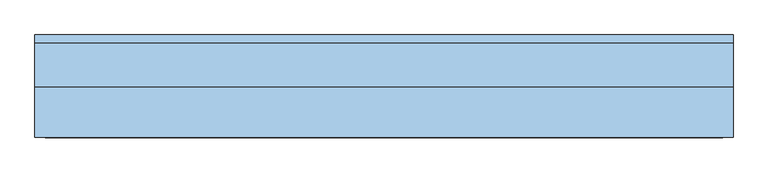
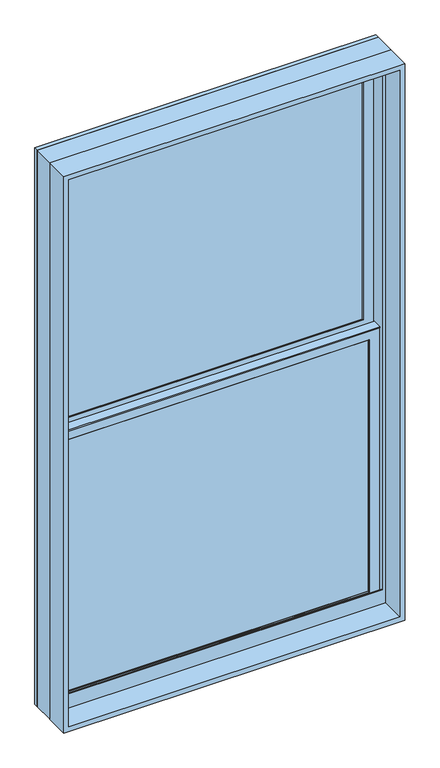
"""IFC4 building model written with IfcOpenShell, lengths in millimetres: window geometry, Window-Double_Hung-Marvin-Essential : ESDH3660."""

from ifc_helpers import new_model, si_unit, frame, origin, place, context, project, spatial, polyline, outline, extrude, faceted_brep, source, transform, mapped, element, save


def window_622c2d66(model_context):
    return source(origin(), model_context, "Body", "SolidModel", [
        extrude(outline(polyline([(166.1583333, 20.6375), (166.1583333, 15.875), (147.1083333, 15.875), (147.1083333, 20.6375), (166.1583333, 20.6375)])), frame((0.0, 0.0, 679.45), z_axis=(0.0, 0.0, 1.0), x_axis=(1.0, 0.0, 0.0)), (0.0, 0.0, 1.0), 831.85),
        extrude(outline(polyline([(-147.1083333, 20.6375), (-147.1083333, 15.875), (-166.1583333, 15.875), (-166.1583333, 20.6375), (-147.1083333, 20.6375)])), frame((0.0, 0.0, 679.45), z_axis=(0.0, 0.0, 1.0), x_axis=(1.0, 0.0, 0.0)), (0.0, 0.0, 1.0), 831.85),
        extrude(outline(polyline([(469.9, 20.6375), (469.9, 15.875), (-469.9, 15.875), (-469.9, 20.6375), (469.9, 20.6375)])), frame((0.0, 0.0, 1085.85), z_axis=(0.0, 0.0, 1.0), x_axis=(1.0, 0.0, 0.0)), (0.0, 0.0, 1.0), 19.05),
        extrude(outline(polyline([(-166.1583333, 46.83125), (-166.1583333, 51.59375), (-147.1083333, 51.59375), (-147.1083333, 46.83125), (-166.1583333, 46.83125)])), frame((0.0, 0.0, 1549.4), z_axis=(0.0, 0.0, 1.0), x_axis=(1.0, 0.0, 0.0)), (0.0, 0.0, 1.0), 831.85),
        extrude(outline(polyline([(147.1083333, 46.83125), (147.1083333, 51.59375), (166.1583333, 51.59375), (166.1583333, 46.83125), (147.1083333, 46.83125)])), frame((0.0, 0.0, 1549.4), z_axis=(0.0, 0.0, 1.0), x_axis=(1.0, 0.0, 0.0)), (0.0, 0.0, 1.0), 831.85),
        extrude(outline(polyline([(-469.9, 46.83125), (-469.9, 51.59375), (469.9, 51.59375), (469.9, 46.83125), (-469.9, 46.83125)])), frame((0.0, 0.0, 1955.8), z_axis=(0.0, 0.0, 1.0), x_axis=(1.0, 0.0, 0.0)), (0.0, 0.0, 1.0), 19.05),
        extrude(outline(polyline([(166.1583333, 20.6375), (147.1083333, 20.6375), (147.1083333, 25.4), (166.1583333, 25.4), (166.1583333, 20.6375)])), frame((0.0, 0.0, 679.45), z_axis=(0.0, 0.0, 1.0), x_axis=(1.0, 0.0, 0.0)), (0.0, 0.0, 1.0), 831.85),
        extrude(outline(polyline([(-147.1083333, 20.6375), (-166.1583333, 20.6375), (-166.1583333, 25.4), (-147.1083333, 25.4), (-147.1083333, 20.6375)])), frame((0.0, 0.0, 679.45), z_axis=(0.0, 0.0, 1.0), x_axis=(1.0, 0.0, 0.0)), (0.0, 0.0, 1.0), 831.85),
        extrude(outline(polyline([(469.9, 20.6375), (-469.9, 20.6375), (-469.9, 25.4), (469.9, 25.4), (469.9, 20.6375)])), frame((0.0, 0.0, 1085.85), z_axis=(0.0, 0.0, 1.0), x_axis=(1.0, 0.0, 0.0)), (0.0, 0.0, 1.0), 19.05),
        extrude(outline(polyline([(-166.1583333, 56.35625), (-147.1083333, 56.35625), (-147.1083333, 51.59375), (-166.1583333, 51.59375), (-166.1583333, 56.35625)])), frame((0.0, 0.0, 1549.4), z_axis=(0.0, 0.0, 1.0), x_axis=(1.0, 0.0, 0.0)), (0.0, 0.0, 1.0), 831.85),
        extrude(outline(polyline([(147.1083333, 56.35625), (166.1583333, 56.35625), (166.1583333, 51.59375), (147.1083333, 51.59375), (147.1083333, 56.35625)])), frame((0.0, 0.0, 1549.4), z_axis=(0.0, 0.0, 1.0), x_axis=(1.0, 0.0, 0.0)), (0.0, 0.0, 1.0), 831.85),
        extrude(outline(polyline([(-469.9, 56.35625), (469.9, 56.35625), (469.9, 51.59375), (-469.9, 51.59375), (-469.9, 56.35625)])), frame((0.0, 0.0, 1955.8), z_axis=(0.0, 0.0, 1.0), x_axis=(1.0, 0.0, 0.0)), (0.0, 0.0, 1.0), 19.05),
        faceted_brep([(-496.8875, 5.6780605, 1541.3351748), (-496.8875, 5.6780605, 1536.7), (496.8875, 5.6780605, 1536.7), (496.8875, 5.6780605, 1541.3351748), (-496.8875, 34.8118605, 1541.3351748), (496.8875, 34.8118605, 1541.3351748), (496.8875, 34.8118605, 1536.7), (-496.8875, 34.8118605, 1536.7), (-496.8875, 30.1625, 1536.7), (-496.8875, 30.1625, 652.4625), (-496.8875, 8.9241104, 652.4625), (-496.8875, 8.9241104, 1536.7), (496.8875, 8.9241104, 1536.7), (496.8875, 30.1625, 1536.7), (496.8875, 8.9241104, 652.4625), (496.8875, 30.1625, 652.4625), (-481.0034752, 11.90625, 1522.4034752), (-481.0034752, 30.1625, 1522.4034752), (481.0034752, 30.1625, 1522.4034752), (481.0034752, 11.90625, 1522.4034752), (-464.34375, 10.4662439, 1505.74375), (-464.34375, 11.90625, 1505.74375), (464.34375, 11.90625, 1505.74375), (464.34375, 10.4662439, 1505.74375), (465.8858834, 8.9241104, 1507.2858834), (-465.8858834, 8.9241104, 1507.2858834), (481.0034752, 30.1625, 668.3465248), (481.0034752, 11.90625, 668.3465248), (464.34375, 11.90625, 685.00625), (464.34375, 10.4662439, 685.00625), (465.8858834, 8.9241104, 683.4641166), (-481.0034752, 30.1625, 668.3465248), (-481.0034752, 11.90625, 668.3465248), (-464.34375, 11.90625, 685.00625), (-464.34375, 10.4662439, 685.00625), (-465.8858834, 8.9241104, 683.4641166)], [[[0, 1, 2, 3]], [[4, 5, 6, 7]], [[1, 0, 4, 7, 8, 9, 10, 11]], [[2, 1, 11, 12]], [[7, 6, 13, 8]], [[3, 2, 12, 14, 15, 13, 6, 5]], [[0, 3, 5, 4]], [[16, 17, 18, 19]], [[20, 21, 22, 23]], [[20, 23, 24, 25]], [[19, 18, 26, 27]], [[23, 22, 28, 29]], [[24, 23, 29, 30]], [[27, 26, 31, 32]], [[29, 28, 33, 34]], [[30, 29, 34, 35]], [[15, 14, 10, 9]], [[15, 9, 8, 13], [18, 17, 31, 26]], [[17, 16, 32, 31]], [[16, 19, 27, 32], [22, 21, 33, 28]], [[21, 20, 34, 33]], [[20, 25, 35, 34]], [[10, 14, 12, 11], [25, 24, 30, 35]]]),
        extrude(outline(polyline([(38.5955581, 1522.4125), (33.5778968, 1522.4125), (33.5778968, 1524.0), (39.9405976, 1524.0), (39.9405976, 1522.4125), (61.515625, 1522.4125), (47.6307501, 1519.0975159), (38.5955581, 1519.0975159), (38.5955581, 1522.4125)])), frame((-496.8875, 0.0, 0.0), z_axis=(1.0, 0.0, 0.0), x_axis=(0.0, 1.0, 0.0)), (0.0, 0.0, 1.0), 993.775),
        faceted_brep([(527.05, 0.0, 622.3), (527.05, 0.0, 2438.4), (-527.05, 0.0, 2438.4), (-527.05, 0.0, 622.3), (500.85625, 0.0, 683.41875), (-500.85625, 0.0, 683.41875), (-500.85625, 0.0, 2412.20625), (500.85625, 0.0, 2412.20625), (500.85625, 3.96875, 622.3), (-500.85625, 3.96875, 622.3), (-500.85625, 3.96875, 683.41875), (500.85625, 3.96875, 683.41875), (-527.05, 65.6828125, 622.3), (-500.85625, 65.6828125, 622.3), (500.85625, 65.6828125, 622.3), (527.05, 65.6828125, 622.3), (-527.05, 65.6828125, 2438.4), (527.05, 65.6828125, 2438.4), (500.85625, 65.6828125, 2412.20625), (-500.85625, 65.6828125, 2412.20625)], [[[0, 1, 2, 3], [4, 5, 6, 7]], [[8, 9, 10, 11]], [[5, 4, 11, 10]], [[0, 3, 12, 13, 9, 8, 14, 15]], [[13, 12, 16, 17, 15, 14, 18, 19]], [[13, 19, 6, 5, 10, 9]], [[7, 6, 19, 18]], [[18, 14, 8, 11, 4, 7]], [[1, 0, 15, 17]], [[2, 1, 17, 16]], [[3, 2, 16, 12]]]),
        faceted_brep([(500.85625, 30.1625, 1530.35), (499.26875, 30.1625, 1530.35), (499.26875, 30.1625, 646.6544613), (500.85625, 30.1625, 646.6544613), (-499.26875, 30.1625, 1530.35), (-500.85625, 30.1625, 1530.35), (-500.85625, 30.1625, 646.6544613), (-499.26875, 30.1625, 646.6544613), (499.26875, 63.5, 1530.35), (500.85625, 63.5, 1530.35), (500.85625, 63.5, 640.1743077), (499.26875, 63.5, 640.1743077), (-500.85625, 63.5, 1530.35), (-499.26875, 63.5, 1530.35), (-499.26875, 63.5, 640.1743077), (-500.85625, 63.5, 640.1743077), (512.1108932, 3.96875, 651.7460105), (512.1108932, 3.96875, 622.3), (512.1108932, 65.6828125, 622.3), (512.1108932, 65.6828125, 639.750012), (-512.1108932, 3.96875, 622.3), (-512.1108932, 3.96875, 651.7460105), (-512.1108932, 65.6828125, 639.750012), (-512.1108932, 65.6828125, 622.3), (512.1108932, 78.58125, 637.2428097), (-512.1108932, 78.58125, 637.2428097), (-510.0971252, 68.2348864, 639.2539391), (-492.13135, 68.2348864, 639.2539391), (-492.13135, 65.6828125, 639.750012), (492.13135, 65.6828125, 639.750012), (492.13135, 68.2348864, 639.2539391), (510.0971252, 68.2348864, 639.2539391), (-527.05, 65.6828125, 622.3), (-527.05, 78.5948249, 622.3), (527.05, 78.5948249, 622.3), (527.05, 65.6828125, 622.3), (-527.05, 78.58125, 2438.4), (527.05, 78.58125, 2438.4), (512.1108932, 78.58125, 2423.4608932), (-512.1108932, 78.58125, 2423.4608932), (-527.05, 65.6828125, 2438.4), (-510.0971252, 68.2348864, 2421.4471252), (510.0971252, 68.2348864, 2421.4471252), (492.13135, 68.2348864, 2403.48135), (-492.13135, 68.2348864, 2403.48135), (-492.13135, 65.6828125, 2403.48135), (492.13135, 65.6828125, 2403.48135), (527.05, 65.6828125, 2438.4)], [[[0, 1, 2, 3]], [[4, 5, 6, 7]], [[8, 9, 10, 11]], [[12, 13, 14, 15]], [[1, 8, 11, 2]], [[9, 0, 3, 10]], [[1, 0, 9, 8]], [[5, 4, 13, 12]], [[5, 12, 15, 6]], [[13, 4, 7, 14]], [[16, 17, 18, 19]], [[20, 21, 22, 23]], [[24, 25, 26, 27, 28, 22, 21, 16, 19, 29, 30, 31], [3, 2, 11, 10], [7, 6, 15, 14]], [[17, 16, 21, 20]], [[17, 20, 23, 32, 33, 34, 35, 18]], [[34, 33, 36, 37], [25, 24, 38, 39]], [[33, 32, 40, 36]], [[39, 41, 26, 25]], [[41, 42, 31, 30, 43, 44, 27, 26]], [[44, 45, 28, 27]], [[40, 32, 23, 22, 28, 45, 46, 29, 19, 18, 35, 47]], [[36, 40, 47, 37]], [[39, 38, 42, 41]], [[44, 43, 46, 45]], [[34, 37, 47, 35]], [[42, 38, 24, 31]], [[46, 43, 30, 29]]]),
        extrude(outline(polyline([(477.04375, 11.90625), (-477.04375, 11.90625), (-477.04375, 15.08125), (477.04375, 15.08125), (477.04375, 11.90625)])), frame((0.0, 0.0, 672.30625), z_axis=(0.0, 0.0, 1.0), x_axis=(1.0, 0.0, 0.0)), (0.0, 0.0, 1.0), 846.1375),
        extrude(outline(polyline([(477.04375, 42.8625), (-477.04375, 42.8625), (-477.04375, 46.0375), (477.04375, 46.0375), (477.04375, 42.8625)])), frame((0.0, 0.0, 1542.25625), z_axis=(0.0, 0.0, 1.0), x_axis=(1.0, 0.0, 0.0)), (0.0, 0.0, 1.0), 846.1375),
        faceted_brep([(-464.34375, 31.194477, 1505.74375), (-465.8858834, 32.7366104, 1507.2858834), (465.8858834, 32.7366104, 1507.2858834), (464.34375, 31.194477, 1505.74375), (-464.34375, 30.1625, 1505.74375), (464.34375, 30.1625, 1505.74375), (-496.8875, 32.7366104, 1538.2875), (-496.8875, 30.1625, 1538.2875), (496.8875, 30.1625, 1538.2875), (496.8875, 32.7366104, 1538.2875), (465.8858834, 32.7366104, 683.4641166), (464.34375, 31.194477, 685.00625), (464.34375, 30.1625, 685.00625), (496.8875, 30.1625, 652.4625), (496.8875, 32.7366104, 652.4625), (-465.8858834, 32.7366104, 683.4641166), (-464.34375, 31.194477, 685.00625), (-464.34375, 30.1625, 685.00625), (-496.8875, 30.1625, 652.4625), (-496.8875, 32.7366104, 652.4625)], [[[0, 1, 2, 3]], [[4, 0, 3, 5]], [[6, 7, 8, 9]], [[3, 2, 10, 11]], [[5, 3, 11, 12]], [[9, 8, 13, 14]], [[11, 10, 15, 16]], [[12, 11, 16, 17]], [[14, 13, 18, 19]], [[9, 14, 19, 6], [1, 15, 10, 2]], [[16, 15, 1, 0]], [[17, 16, 0, 4]], [[7, 18, 13, 8], [5, 12, 17, 4]], [[19, 18, 7, 6]]]),
        faceted_brep([(-481.0034752, 42.8625, 2392.3534752), (-481.0034752, 61.11875, 2392.3534752), (481.0034752, 61.11875, 2392.3534752), (481.0034752, 42.8625, 2392.3534752), (-464.34375, 41.4224939, 2375.69375), (-464.34375, 42.8625, 2375.69375), (464.34375, 42.8625, 2375.69375), (464.34375, 41.4224939, 2375.69375), (-465.8858834, 39.8803604, 2377.2358834), (465.8858834, 39.8803604, 2377.2358834), (-496.8875, 61.11875, 2408.2375), (-496.8875, 39.8803604, 2408.2375), (496.8875, 39.8803604, 2408.2375), (496.8875, 61.11875, 2408.2375), (481.0034752, 61.11875, 1538.2965248), (481.0034752, 42.8625, 1538.2965248), (464.34375, 42.8625, 1554.95625), (464.34375, 41.4224939, 1554.95625), (465.8858834, 39.8803604, 1553.4141166), (496.8875, 39.8803604, 1522.4125), (496.8875, 61.11875, 1522.4125), (-481.0034752, 61.11875, 1538.2965248), (-481.0034752, 42.8625, 1538.2965248), (-464.34375, 42.8625, 1554.95625), (-464.34375, 41.4224939, 1554.95625), (-465.8858834, 39.8803604, 1553.4141166), (-496.8875, 39.8803604, 1522.4125), (-496.8875, 61.11875, 1522.4125)], [[[0, 1, 2, 3]], [[4, 5, 6, 7]], [[8, 4, 7, 9]], [[10, 11, 12, 13]], [[3, 2, 14, 15]], [[7, 6, 16, 17]], [[9, 7, 17, 18]], [[13, 12, 19, 20]], [[15, 14, 21, 22]], [[17, 16, 23, 24]], [[18, 17, 24, 25]], [[20, 19, 26, 27]], [[13, 20, 27, 10], [1, 21, 14, 2]], [[22, 21, 1, 0]], [[3, 15, 22, 0], [5, 23, 16, 6]], [[24, 23, 5, 4]], [[25, 24, 4, 8]], [[11, 26, 19, 12], [9, 18, 25, 8]], [[27, 26, 11, 10]]]),
        faceted_brep([(-496.8875, 61.11875, 1522.4125), (-496.8875, 63.6928604, 1522.4125), (496.8875, 63.6928604, 1522.4125), (496.8875, 61.11875, 1522.4125), (-464.34375, 62.150727, 1554.95625), (-464.34375, 61.11875, 1554.95625), (464.34375, 61.11875, 1554.95625), (464.34375, 62.150727, 1554.95625), (-465.8858834, 63.6928604, 1553.4141166), (465.8858834, 63.6928604, 1553.4141166), (496.8875, 63.6928604, 2408.2375), (496.8875, 61.11875, 2408.2375), (464.34375, 61.11875, 2375.69375), (464.34375, 62.150727, 2375.69375), (465.8858834, 63.6928604, 2377.2358834), (-496.8875, 63.6928604, 2408.2375), (-496.8875, 61.11875, 2408.2375), (-464.34375, 61.11875, 2375.69375), (-464.34375, 62.150727, 2375.69375), (-465.8858834, 63.6928604, 2377.2358834)], [[[0, 1, 2, 3]], [[4, 5, 6, 7]], [[8, 4, 7, 9]], [[3, 2, 10, 11]], [[7, 6, 12, 13]], [[9, 7, 13, 14]], [[11, 10, 15, 16]], [[13, 12, 17, 18]], [[14, 13, 18, 19]], [[16, 15, 1, 0]], [[3, 11, 16, 0], [5, 17, 12, 6]], [[18, 17, 5, 4]], [[19, 18, 4, 8]], [[1, 15, 10, 2], [9, 14, 19, 8]]]),
        extrude(outline(polyline([(477.04375, 26.19375), (-477.04375, 26.19375), (-477.04375, 30.1625), (477.04375, 30.1625), (477.04375, 26.19375)])), frame((0.0, 0.0, 672.30625), z_axis=(0.0, 0.0, 1.0), x_axis=(1.0, 0.0, 0.0)), (0.0, 0.0, 1.0), 846.1375),
        extrude(outline(polyline([(477.04375, 57.15), (-477.04375, 57.15), (-477.04375, 61.11875), (477.04375, 61.11875), (477.04375, 57.15)])), frame((0.0, 0.0, 1542.25625), z_axis=(0.0, 0.0, 1.0), x_axis=(1.0, 0.0, 0.0)), (0.0, 0.0, 1.0), 846.1375),
        extrude(outline(polyline([(2438.4, 527.05), (2438.4, -527.05), (622.3, -527.05), (622.3, 527.05), (2438.4, 527.05)]), holes=[polyline([(2422.525, 511.175), (638.175, 511.175), (638.175, -511.175), (2422.525, -511.175), (2422.525, 511.175)])]), frame((0.0, -76.2, 0.0), z_axis=(0.0, 1.0, 0.0), x_axis=(0.0, 0.0, 1.0)), (0.0, 0.0, 1.0), 75.40625),
    ])


if __name__ == "__main__":
    model = new_model("IFC4")
    model_context = context("Model", 3, world=origin())
    ifc_project = project(units=[si_unit("LENGTHUNIT", "METRE", prefix="MILLI")], contexts=[model_context])
    site = spatial("IfcSite", under=ifc_project)
    building = spatial("IfcBuilding", under=site)
    placement = place(None, origin())
    window_shape = window_622c2d66(model_context)
    element("IfcWindow", 1, ObjectType="Window-Double_Hung-Marvin-Essential : ESDH3660", at=placement, inside=building, context=model_context, shape_type="MappedRepresentation", body=[
        mapped(window_shape, transform((0.0, 0.0, 0.0), x_axis=(1.0, 0.0, 0.0), y_axis=(0.0, 1.0, 0.0), z_axis=(0.0, 0.0, 1.0))),
    ])
    save(model, "model.ifc")

# Revit data of these elements
# Type "Window-Double_Hung-Marvin-Essential : ESDH3660"
#   Type Mark = "80"
#   Window Type = "Essential Double Hung"
#   Product data url = "https://bimobject.com/marvin-windows-and-doors/product/marvin-dhwau"
#   Product Guid = "c4a96547-874c-4385-91dc-a058adc19d98"
#   Frame = "All Ultrex"
#   Egress Window = "Yes"
#   URL = "www.marvin.com"
#   Model = "ESDH3660"
#   Manufacturer = "Marvin Windows and Doors"
#   Label Egress = "EGRESS WDW"
#   Glass Type = "IG Low E II with Argon"
#   Design Pressure = "DP30"
#   Description = "4272 DBHG"
#   Analytic Construction = "<None>"
#   Prairie Corner Width = 0' - 4"
#   Prairie Corner Height = 0' - 4"
#   Egress Width = 3' - 2 9/16"
#   Egress Height = 2' - 7 27/128"
#   Rough Width = 3' - 6"
#   Rough Height = 6' - 0"
#   Nominal Width = 3' - 6"
#   Nominal Height = 6' - 0"
#   Inset to Installation Flange [instance default] = 0' - 1"
#   Height = 5' - 11 1/2"
#   Egress Area = 8.35814 SF
#   Default Head Height = 8' - 0"
#   Width = 3' - 5 1/2"
#   Daylight Area = 16.4087 SF
#   DLO Width = 3' - 0 9/16"
#   DLO Height = 2' - 8 5/16"
#   Muntins Top Sash = yes
#   Lites Wide Top Sash = 3
#   Lites Wide Bottom Sash = 3
#   Lites High Top Sash = 2
#   Lites High Bottom Sash = 2
#   Lite Cut Prairie 9 = no
#   Lite Cut HV Grid = yes
#   Muntins Bottom Sash = yes
#   Label Visibility = no
#   Jamb Extension Visibility = yes
#   Edition number = 1
#   Interior Material = Ultrex-Marvin-Stonewhite
#   Glazing Material = Glass-Marvin-IG Low E II with Argon
#   Cladding Material = Ultrex-Marvin-Pebblegray
#   Wall Closure = (empty or 0)
#   Assembly Code = ""
# Element 1 (IfcWindow, "Window-Double_Hung-Marvin-Essential : ESDH3660")
#   Materials on its faces: "Ultrex-Marvin-Pebblegray", "Ultrex-Marvin-Stonewhite", "Glass-Marvin-IG Low E II with Argon"
# Materials
#   "Ultrex-Marvin-Stonewhite": class "Paint", colour RGB 250 251 245, transparency 0
#   "Glass-Marvin-IG Low E II with Argon": class "Glass", colour RGB 0 128 192, transparency 0.85
#   "Ultrex-Marvin-Pebblegray": class "Paint", colour RGB 189 185 173, transparency 0
